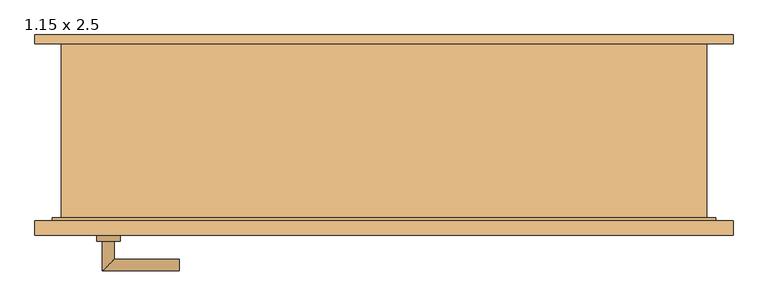
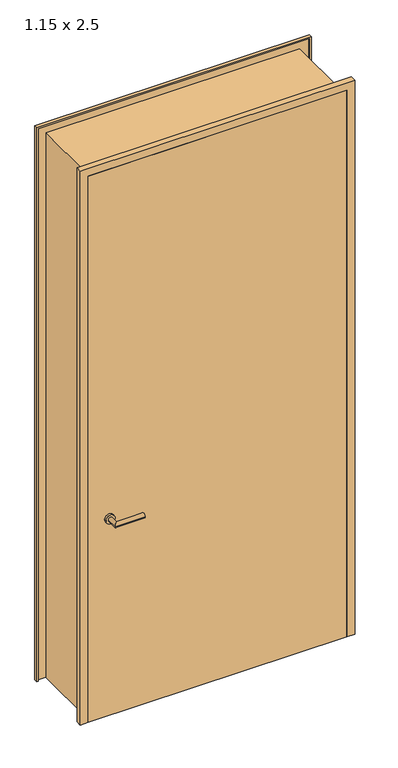
"""IFC4 building model written with IfcOpenShell, lengths in millimetres: door geometry, Drehflügel 1-flg - Stahlzarge : 1.15 x 2.5."""

import ifcopenshell
import ifcopenshell.guid

model = None  # the IFC model being written
_history = None  # IfcOwnerHistory: only IFC2X3 demands one
_inside = {}  # id of a spatial element -> (the spatial element, [elements in it])
_under = {}  # id of a project, library or spatial element -> (it, [spatial elements below it])
_declared = {}  # id of a project -> (the project, [libraries it declares])
_typed = {}  # id of a type object -> (the type object, [elements of that type])
_made_of = {}  # id of a material, layer set ... -> (it, [elements and type objects made of it])


def new_model(schema):
    """Start an empty IFC model of exactly this schema.

    Asked for "IFC4X3", IfcOpenShell would pick the latest addendum, in which some entities
    have other attributes; the version numbers below select the first issue.
    IFC2X3 requires an IfcOwnerHistory on every rooted entity: one is made here for all.
    """
    global model, _history
    if schema == "IFC4X3":
        model = ifcopenshell.file(schema_version=(4, 3, 0, 0))
    else:
        model = ifcopenshell.file(schema=schema)
    _inside.clear()
    _under.clear()
    _declared.clear()
    _typed.clear()
    _made_of.clear()
    _history = None
    if model.schema == "IFC2X3":
        org = make("IfcOrganization", Name="unknown")
        user = make(
            "IfcPersonAndOrganization",
            ThePerson=make("IfcPerson", FamilyName="unknown"),
            TheOrganization=org,
        )
        app = make(
            "IfcApplication",
            ApplicationDeveloper=org,
            Version="unknown",
            ApplicationFullName="unknown",
            ApplicationIdentifier="unknown",
        )
        _history = make(
            "IfcOwnerHistory",
            OwningUser=user,
            OwningApplication=app,
            ChangeAction="ADDED",
            CreationDate=0,
        )
    return model


def make(cls, **values):
    """One entity of the class cls with the attributes given. An attribute that is None is left unset."""
    return model.create_entity(
        cls, **{name: value for name, value in values.items() if value is not None}
    )


def rooted(cls, **values):
    """An entity with a GlobalId (a new one), such as an element, a storey or a relation."""
    return make(cls, GlobalId=ifcopenshell.guid.new(), OwnerHistory=_history, **values)


def si_unit(unit_type, name, prefix=None):
    """IfcSIUnit, for example si_unit("LENGTHUNIT", "METRE", prefix="MILLI")."""
    return make("IfcSIUnit", UnitType=unit_type, Prefix=prefix, Name=name)


def assignment(units):
    """IfcUnitAssignment: the units of a project."""
    return None if units is None else make("IfcUnitAssignment", Units=units)


def point(xyz):
    """IfcCartesianPoint."""
    return None if xyz is None else make("IfcCartesianPoint", Coordinates=xyz)


def direction(xyz):
    """IfcDirection."""
    return None if xyz is None else make("IfcDirection", DirectionRatios=xyz)


def frame(location, z_axis=None, x_axis=None):
    """IfcAxis2Placement3D, a coordinate frame: its origin and axes. An axis left out is left unset."""
    return make(
        "IfcAxis2Placement3D",
        Location=point(location),
        Axis=direction(z_axis),
        RefDirection=direction(x_axis),
    )


def frame_2d(location, x_axis=None):
    """IfcAxis2Placement2D, a coordinate frame in the plane: its origin and x axis."""
    return make(
        "IfcAxis2Placement2D", Location=point(location), RefDirection=direction(x_axis)
    )


def origin():
    """The frame at (0, 0, 0) with its axes left unset."""
    return frame((0.0, 0.0, 0.0))


def place(relative_to, where):
    """IfcLocalPlacement: puts the frame where relative to a parent placement (None: the world)."""
    return make(
        "IfcLocalPlacement", PlacementRelTo=relative_to, RelativePlacement=where
    )


def context(
    kind, dimensions, precision=None, world=None, true_north=None, identifier=None
):
    """IfcGeometricRepresentationContext, for example the 3D "Model" context."""
    return make(
        "IfcGeometricRepresentationContext",
        ContextIdentifier=identifier,
        ContextType=kind,
        CoordinateSpaceDimension=dimensions,
        Precision=precision,
        WorldCoordinateSystem=world,
        TrueNorth=true_north,
    )


def project(units=None, contexts=None):
    """IfcProject with its units and contexts."""
    return rooted(
        "IfcProject",
        Name="project",
        RepresentationContexts=contexts,
        UnitsInContext=assignment(units),
    )


def spatial(cls, under=None, at=None, **own):
    """A site, building, storey or space (cls), placed at a placement, below another one or the project."""
    s = rooted(cls, ObjectPlacement=at, **own)
    if under is not None:
        _under.setdefault(under.id(), (under, []))[1].append(s)
    return s


def polyline(points):
    """IfcPolyline through the points."""
    return make("IfcPolyline", Points=[point(p) for p in points])


def circle_curve(where, radius):
    """IfcCircle in the frame where."""
    return make("IfcCircle", Position=where, Radius=radius)


def ellipse_curve(where, semi_axis1, semi_axis2):
    """IfcEllipse in the frame where."""
    return make(
        "IfcEllipse", Position=where, SemiAxis1=semi_axis1, SemiAxis2=semi_axis2
    )


def trimmed(basis, trim1, trim2, sense, master):
    """IfcTrimmedCurve: the piece of a basis curve between two trims."""
    return make(
        "IfcTrimmedCurve",
        BasisCurve=basis,
        Trim1=trim1,
        Trim2=trim2,
        SenseAgreement=sense,
        MasterRepresentation=master,
    )


def segment(curve, same_sense, transition):
    """IfcCompositeCurveSegment."""
    return make(
        "IfcCompositeCurveSegment",
        Transition=transition,
        SameSense=same_sense,
        ParentCurve=curve,
    )


def composite_curve(segments, self_intersect=None):
    """IfcCompositeCurve: segments joined end to end."""
    return make("IfcCompositeCurve", Segments=segments, SelfIntersect=self_intersect)


def outline(outer, holes=None, kind="AREA"):
    """IfcArbitraryClosedProfileDef: a profile drawn as a closed curve; with holes, ...WithVoids."""
    if holes is None:
        return make("IfcArbitraryClosedProfileDef", ProfileType=kind, OuterCurve=outer)
    return make(
        "IfcArbitraryProfileDefWithVoids",
        ProfileType=kind,
        OuterCurve=outer,
        InnerCurves=holes,
    )


def extrude(swept, where, along, depth):
    """IfcExtrudedAreaSolid: the profile swept, set in the frame where, extruded along a direction by depth."""
    return make(
        "IfcExtrudedAreaSolid",
        SweptArea=swept,
        Position=where,
        ExtrudedDirection=direction(along),
        Depth=depth,
    )


def faces_of(points, faces, orient=None, outer=None):
    """IfcFace entities. A face is a list of loops; a loop is a list of indices into points, from 0.

    orient and outer hold one flag for each loop. By default every Orientation is true, the
    first loop of a face is its IfcFaceOuterBound and the others are IfcFaceBound.
    """
    made = []
    for i, loops in enumerate(faces):
        bounds = []
        for j, loop in enumerate(loops):
            is_outer = j == 0 if outer is None else outer[i][j]
            bounds.append(
                make(
                    "IfcFaceOuterBound" if is_outer else "IfcFaceBound",
                    Bound=make("IfcPolyLoop", Polygon=[points[k] for k in loop]),
                    Orientation=True if orient is None else orient[i][j],
                )
            )
        made.append(make("IfcFace", Bounds=bounds))
    return made


def faceted_brep(points, faces, orient=None, outer=None, voids=None):
    """IfcFacetedBrep: a solid bounded by flat faces; with voids (closed shells), ...WithVoids."""
    shared = [point(p) for p in points]
    hull = make("IfcClosedShell", CfsFaces=faces_of(shared, faces, orient, outer))
    if voids is None:
        return make("IfcFacetedBrep", Outer=hull)
    return make(
        "IfcFacetedBrepWithVoids",
        Outer=hull,
        Voids=[
            make(cls, CfsFaces=faces_of(shared, fs, o, b)) for cls, fs, o, b in voids
        ],
    )


def shape(context_of_items, identifier, shape_type, items):
    """IfcShapeRepresentation: the items that make up one representation, for example the "Body"."""
    return make(
        "IfcShapeRepresentation",
        ContextOfItems=context_of_items,
        RepresentationIdentifier=identifier,
        RepresentationType=shape_type,
        Items=items,
    )


def source(mapping_origin, context_of_items, identifier, shape_type, items):
    """IfcRepresentationMap: a shape defined once, which mapped items show again and again."""
    return make(
        "IfcRepresentationMap",
        MappingOrigin=mapping_origin,
        MappedRepresentation=shape(context_of_items, identifier, shape_type, items),
    )


def transform(
    local_origin,
    x_axis=None,
    y_axis=None,
    z_axis=None,
    scale=None,
    scale2=None,
    scale3=None,
    uniform=True,
):
    """IfcCartesianTransformationOperator3D, or its non-uniform kind. x_axis, y_axis, z_axis: its Axis1, 2, 3."""
    if uniform:
        return make(
            "IfcCartesianTransformationOperator3D",
            Axis1=direction(x_axis),
            Axis2=direction(y_axis),
            LocalOrigin=point(local_origin),
            Scale=scale,
            Axis3=direction(z_axis),
        )
    return make(
        "IfcCartesianTransformationOperator3DnonUniform",
        Axis1=direction(x_axis),
        Axis2=direction(y_axis),
        LocalOrigin=point(local_origin),
        Scale=scale,
        Axis3=direction(z_axis),
        Scale2=scale2,
        Scale3=scale3,
    )


def mapped(mapping_source, mapping_target):
    """IfcMappedItem: shows the shape of a source again, moved by a transform."""
    return make(
        "IfcMappedItem", MappingSource=mapping_source, MappingTarget=mapping_target
    )


def made_of(thing, what):
    """Note that an element or type object is made of a material, layer set ...; save() writes the relation."""
    if what is not None:
        _made_of.setdefault(what.id(), (what, []))[1].append(thing)
    return thing


def element(
    cls,
    number,
    at=None,
    inside=None,
    cuts=None,
    type_object=None,
    material=None,
    context=None,
    identifier="Body",
    shape_type=None,
    held_by="IfcProductDefinitionShape",
    body=None,
    shapes=None,
    **own,
):
    """One element of the class cls, such as IfcWall. Its Tag is "e" and its number.

    at: its placement. inside: the storey or other place that contains it. cuts: it is an
    opening in that element (IfcRelVoidsElement). A single representation is given by context,
    identifier, shape_type and body (its items); several are given by shapes. held_by: the class
    of the entity that holds the representations. save() writes the other relations.
    """
    e = rooted(cls, Tag="e%d" % number, ObjectPlacement=at, **own)
    if body is not None:
        shapes = [shape(context, identifier, shape_type, body)]
    if shapes is not None:
        e.Representation = make(held_by, Representations=shapes)
    if inside is not None:
        _inside.setdefault(inside.id(), (inside, []))[1].append(e)
    if cuts is not None:
        rooted(
            "IfcRelVoidsElement", RelatingBuildingElement=cuts, RelatedOpeningElement=e
        )
    if type_object is not None:
        _typed.setdefault(type_object.id(), (type_object, []))[1].append(e)
    return made_of(e, material)


def aggregate(whole, parts):
    """IfcRelAggregates: a whole, such as a stair, and the parts it consists of."""
    return rooted("IfcRelAggregates", RelatingObject=whole, RelatedObjects=parts)


def save(model, path):
    """Write the relations noted so far, then the file.

    IfcRelAggregates (storeys below a building ...), IfcRelContainedInSpatialStructure (elements
    in a storey), IfcRelDefinesByType, IfcRelAssociatesMaterial and IfcRelDeclares: one each for
    every whole, place, type object, material and project.
    """
    for whole, parts in _under.values():
        aggregate(whole, parts)
    for where, things in _inside.values():
        rooted(
            "IfcRelContainedInSpatialStructure",
            RelatedElements=things,
            RelatingStructure=where,
        )
    for kind, things in _typed.values():
        rooted("IfcRelDefinesByType", RelatedObjects=things, RelatingType=kind)
    for what, things in _made_of.values():
        rooted("IfcRelAssociatesMaterial", RelatedObjects=things, RelatingMaterial=what)
    for by, libraries in _declared.values():
        rooted("IfcRelDeclares", RelatingContext=by, RelatedDefinitions=libraries)
    model.write(path)


def plane_surface(at):
    """IfcPlane: the flat surface through the origin of the frame at, square to its z axis."""
    return make("IfcPlane", Position=at)


def cylinder_surface(at, radius):
    """IfcCylindricalSurface: all points at the distance radius from the z axis of the frame at."""
    return make("IfcCylindricalSurface", Position=at, Radius=radius)


def advanced_brep(points, edges, surfaces, faces):
    """IfcAdvancedBrep: a solid bounded by faces that lie on surfaces and meet in shared edges.

    An edge is (start, end): straight between two places in points (the first is 0);
    or (start, end, curve); or (start, end, curve, False) where it runs against its curve.
    A face is (place in surfaces, loops), or (place, loops, False) where it looks against
    its surface's normal. A loop lists edges by number (the first is 1), with a minus sign
    where the edge is run from its end to its start. The first loop is the outer one.
    """
    corners = [point(p) for p in points]
    vertices = [make("IfcVertexPoint", VertexGeometry=c) for c in corners]
    made = []
    for start, end, *more in edges:
        made.append(
            make(
                "IfcEdgeCurve",
                EdgeStart=vertices[start],
                EdgeEnd=vertices[end],
                EdgeGeometry=more[0] if more else make("IfcPolyline", Points=[corners[start], corners[end]]),
                SameSense=more[1] if len(more) > 1 else True,
            )
        )
    hull = []
    for where, loops, *sense in faces:
        bounds = []
        for j, loop in enumerate(loops):
            ring = [make("IfcOrientedEdge", EdgeElement=made[abs(k) - 1], Orientation=k > 0) for k in loop]
            bounds.append(
                make(
                    "IfcFaceOuterBound" if j == 0 else "IfcFaceBound",
                    Bound=make("IfcEdgeLoop", EdgeList=ring),
                    Orientation=True,
                )
            )
        hull.append(make("IfcAdvancedFace", Bounds=bounds, FaceSurface=surfaces[where], SameSense=sense[0] if sense else True))
    return make("IfcAdvancedBrep", Outer=make("IfcClosedShell", CfsFaces=hull))


def door_1_15_x_2_5_3822d9ce(model_context):
    return source(origin(), model_context, "Body", "SolidModel", [
        advanced_brep(
        [(-477.5, -139.4346141, 901.0), (-457.5, -139.4346141, 901.0), (-457.5, -89.4346141, 901.0), (-477.5, -69.4346141, 901.0), (-347.5, -69.4346141, 901.0), (-347.5, -89.4346141, 901.0)],
        [
            (0, 1, circle_curve(frame((-467.5, -139.4346141, 901.0), z_axis=(0.0, -1.0, 0.0), x_axis=(1.0, 0.0, 0.0)), 10.0)),
            (1, 0, circle_curve(frame((-467.5, -139.4346141, 901.0), z_axis=(0.0, -1.0, 0.0), x_axis=(1.0, 0.0, 0.0)), 10.0)),
            (1, 2),
            (2, 3, ellipse_curve(frame((-467.5, -79.4346141, 901.0), z_axis=(-0.7071067811865385, -0.7071067811865565, 0.0), x_axis=(0.7071067811865563, -0.7071067811865386, 0.0)), 14.1421356, 10.0)),
            (3, 0),
            (3, 2, ellipse_curve(frame((-467.5, -79.4346141, 901.0), z_axis=(-0.7071067811865385, -0.7071067811865565, 0.0), x_axis=(0.7071067811865563, -0.7071067811865386, 0.0)), 14.1421356, 10.0)),
            (4, 5, circle_curve(frame((-347.5, -79.4346141, 901.0), z_axis=(1.0, 0.0, 0.0), x_axis=(0.0, -1.0, 0.0)), 10.0)),
            (5, 4, circle_curve(frame((-347.5, -79.4346141, 901.0), z_axis=(1.0, 0.0, 0.0), x_axis=(0.0, -1.0, 0.0)), 10.0)),
            (2, 5),
            (4, 3),
        ],
        [
            plane_surface(frame((-467.5, -139.4346141, -386.7526403), z_axis=(0.0, -1.0, 0.0), x_axis=(0.0, 0.0, 1.0))),
            cylinder_surface(frame((-467.5, -139.4346141, 901.0), z_axis=(0.0, -1.0, 0.0), x_axis=(1.0, 0.0, 0.0)), 10.0),
            plane_surface(frame((-347.5, -79.4346141, -386.7526403), z_axis=(1.0, 0.0, 0.0), x_axis=(0.0, 0.0, 1.0))),
            cylinder_surface(frame((-467.5, -79.4346141, 901.0), z_axis=(-1.0, 0.0, 0.0), x_axis=(0.0, -1.0, 0.0)), 10.0),
        ],
        [
            (0, [[1, 2]]),
            (1, [[3, 4, 5, -2]]),
            (1, [[-5, 6, -3, -1]]),
            (2, [[7, 8]]),
            (3, [[9, -7, 10, -4]]),
            (3, [[-10, -8, -9, -6]]),
        ],
    ),
        advanced_brep(
        [(-457.5, -199.4346141, 901.0), (-477.5, -199.4346141, 901.0), (-477.5, -249.4346141, 901.0), (-457.5, -229.4346141, 901.0), (-347.5, -229.4346141, 901.0), (-347.5, -249.4346141, 901.0)],
        [
            (0, 1, circle_curve(frame((-467.5, -199.4346141, 901.0), z_axis=(0.0, 1.0, 0.0), x_axis=(-1.0, 0.0, 0.0)), 10.0)),
            (1, 0, circle_curve(frame((-467.5, -199.4346141, 901.0), z_axis=(0.0, 1.0, 0.0), x_axis=(-1.0, 0.0, 0.0)), 10.0)),
            (1, 2),
            (2, 3, ellipse_curve(frame((-467.5, -239.4346141, 901.0), z_axis=(-0.7071067811865475, 0.7071067811865475, 0.0), x_axis=(0.7071067811865474, 0.7071067811865476, 0.0)), 14.1421356, 10.0)),
            (3, 0),
            (3, 2, ellipse_curve(frame((-467.5, -239.4346141, 901.0), z_axis=(-0.7071067811865475, 0.7071067811865475, 0.0), x_axis=(0.7071067811865474, 0.7071067811865476, 0.0)), 14.1421356, 10.0)),
            (4, 5, circle_curve(frame((-347.5, -239.4346141, 901.0), z_axis=(1.0, 0.0, 0.0), x_axis=(0.0, -1.0, 0.0)), 10.0)),
            (5, 4, circle_curve(frame((-347.5, -239.4346141, 901.0), z_axis=(1.0, 0.0, 0.0), x_axis=(0.0, -1.0, 0.0)), 10.0)),
            (2, 5),
            (4, 3),
        ],
        [
            plane_surface(frame((-467.5, -199.4346141, -386.7526403), z_axis=(0.0, 1.0, 0.0), x_axis=(0.0, 0.0, 1.0))),
            cylinder_surface(frame((-467.5, -199.4346141, 901.0), z_axis=(0.0, 1.0, 0.0), x_axis=(-1.0, 0.0, 0.0)), 10.0),
            plane_surface(frame((-347.5, -239.4346141, -386.7526403), z_axis=(1.0, 0.0, 0.0), x_axis=(0.0, 0.0, 1.0))),
            cylinder_surface(frame((-467.5, -239.4346141, 901.0), z_axis=(-1.0, 0.0, 0.0), x_axis=(0.0, -1.0, 0.0)), 10.0),
        ],
        [
            (0, [[1, 2]]),
            (1, [[3, 4, 5, -2]]),
            (1, [[-5, 6, -3, -1]]),
            (2, [[7, 8]]),
            (3, [[9, -7, 10, -4]]),
            (3, [[-10, -8, -9, -6]]),
        ],
    ),
        extrude(outline(composite_curve([segment(trimmed(circle_curve(frame_2d((901.0, -467.5)), 20.0), [point((901.0, -487.5))], [point((901.0, -447.5))], False, "CARTESIAN"), True, "CONTINUOUS"), segment(trimmed(circle_curve(frame_2d((901.0, -467.5)), 20.0), [point((901.0, -447.5))], [point((901.0, -487.5))], False, "CARTESIAN"), True, "CONTINUOUS")], self_intersect=False)), frame((0.0, -139.4346141, 0.0), z_axis=(0.0, 1.0, 0.0), x_axis=(0.0, 0.0, 1.0)), (0.0, 0.0, 1.0), 10.0),
        extrude(outline(composite_curve([segment(trimmed(circle_curve(frame_2d((901.0, -467.5)), 20.0), [point((901.0, -487.5))], [point((901.0, -447.5))], False, "CARTESIAN"), True, "CONTINUOUS"), segment(trimmed(circle_curve(frame_2d((901.0, -467.5)), 20.0), [point((901.0, -447.5))], [point((901.0, -487.5))], False, "CARTESIAN"), True, "CONTINUOUS")], self_intersect=False)), frame((0.0, -199.4346141, 0.0), z_axis=(0.0, 1.0, 0.0), x_axis=(0.0, 0.0, 1.0)), (0.0, 0.0, 1.0), 10.0),
        extrude(outline(polyline([(557.5, -164.4346141), (557.5, -189.4346141), (-557.5, -189.4346141), (-557.5, -164.4346141), (557.5, -164.4346141)])), frame((0.0, 0.0, 1.0), z_axis=(0.0, 0.0, 1.0), x_axis=(1.0, 0.0, 0.0)), (0.0, 0.0, 1.0), 2490.0),
        faceted_brep([(591.9603207, 150.5653859, 1.0), (591.9603207, 135.5653859, 1.0), (586.9603207, 135.5653859, 1.0), (586.9603207, 145.5653859, 1.0), (547.5, 145.5653859, 1.0), (547.5, -159.4346141, 1.0), (562.5, -159.4346141, 1.0), (562.5, -184.4346141, 1.0), (586.9603207, -184.4346141, 1.0), (586.9603207, -164.4346141, 1.0), (591.9603207, -164.4346141, 1.0), (591.9603207, -189.4346141, 1.0), (557.5, -189.4346141, 1.0), (557.5, -164.4346141, 1.0), (542.5, -164.4346141, 1.0), (542.5, 150.5653859, 1.0), (542.5, 150.5653859, 2476.0), (-542.5, 150.5653859, 2476.0), (-542.5, 150.5653859, 1.0), (-591.9603207, 150.5653859, 1.0), (-591.9603207, 150.5653859, 2525.4603207), (591.9603207, 150.5653859, 2525.4603207), (542.5, -164.4346141, 2476.0), (557.5, -164.4346141, 2491.0), (-557.5, -164.4346141, 2491.0), (-557.5, -164.4346141, 1.0), (-542.5, -164.4346141, 1.0), (-542.5, -164.4346141, 2476.0), (557.5, -189.4346141, 2491.0), (591.9603207, -189.4346141, 2525.4603207), (-591.9603207, -189.4346141, 2525.4603207), (-591.9603207, -189.4346141, 1.0), (-557.5, -189.4346141, 1.0), (-557.5, -189.4346141, 2491.0), (591.9603207, -164.4346141, 2525.4603207), (586.9603207, -164.4346141, 2520.4603207), (-586.9603207, -164.4346141, 2520.4603207), (-586.9603207, -164.4346141, 1.0), (-591.9603207, -164.4346141, 1.0), (-591.9603207, -164.4346141, 2525.4603207), (586.9603207, -184.4346141, 2520.4603207), (562.5, -184.4346141, 2496.0), (-562.5, -184.4346141, 2496.0), (-562.5, -184.4346141, 1.0), (-586.9603207, -184.4346141, 1.0), (-586.9603207, -184.4346141, 2520.4603207), (562.5, -159.4346141, 2496.0), (547.5, -159.4346141, 2481.0), (-547.5, -159.4346141, 2481.0), (-547.5, -159.4346141, 1.0), (-562.5, -159.4346141, 1.0), (-562.5, -159.4346141, 2496.0), (547.5, 145.5653859, 2481.0), (586.9603207, 145.5653859, 2520.4603207), (-586.9603207, 145.5653859, 2520.4603207), (-586.9603207, 145.5653859, 1.0), (-547.5, 145.5653859, 1.0), (-547.5, 145.5653859, 2481.0), (586.9603207, 135.5653859, 2520.4603207), (591.9603207, 135.5653859, 2525.4603207), (-591.9603207, 135.5653859, 2525.4603207), (-591.9603207, 135.5653859, 1.0), (-586.9603207, 135.5653859, 1.0), (-586.9603207, 135.5653859, 2520.4603207)], [[[0, 1, 2, 3, 4, 5, 6, 7, 8, 9, 10, 11, 12, 13, 14, 15]], [[15, 16, 17, 18, 19, 20, 21, 0]], [[14, 22, 16, 15]], [[13, 23, 24, 25, 26, 27, 22, 14]], [[12, 28, 23, 13]], [[11, 29, 30, 31, 32, 33, 28, 12]], [[10, 34, 29, 11]], [[9, 35, 36, 37, 38, 39, 34, 10]], [[8, 40, 35, 9]], [[7, 41, 42, 43, 44, 45, 40, 8]], [[6, 46, 41, 7]], [[5, 47, 48, 49, 50, 51, 46, 6]], [[4, 52, 47, 5]], [[3, 53, 54, 55, 56, 57, 52, 4]], [[2, 58, 53, 3]], [[1, 59, 60, 61, 62, 63, 58, 2]], [[0, 21, 59, 1]], [[20, 19, 61, 60]], [[19, 18, 26, 25, 32, 31, 38, 37, 44, 43, 50, 49, 56, 55, 62, 61]], [[27, 26, 18, 17]], [[33, 32, 25, 24]], [[39, 38, 31, 30]], [[45, 44, 37, 36]], [[51, 50, 43, 42]], [[57, 56, 49, 48]], [[63, 62, 55, 54]], [[22, 27, 17, 16]], [[28, 33, 24, 23]], [[34, 39, 30, 29]], [[40, 45, 36, 35]], [[46, 51, 42, 41]], [[52, 57, 48, 47]], [[58, 63, 54, 53]], [[21, 20, 60, 59]]]),
    ])


if __name__ == "__main__":
    model = new_model("IFC4")
    model_context = context("Model", 3, world=origin())
    ifc_project = project(units=[si_unit("LENGTHUNIT", "METRE", prefix="MILLI")], contexts=[model_context])
    site = spatial("IfcSite", under=ifc_project)
    building = spatial("IfcBuilding", under=site)
    placement = place(None, origin())
    door_1_15_x_2_5_shape = door_1_15_x_2_5_3822d9ce(model_context)
    element("IfcDoor", 1, ObjectType="Drehflügel 1-flg - Stahlzarge : 1.15 x 2.5", at=placement, inside=building, context=model_context, shape_type="MappedRepresentation", body=[
        mapped(door_1_15_x_2_5_shape, transform((0.0, 0.0, 0.0), x_axis=(1.0, 0.0, 0.0), y_axis=(0.0, 1.0, 0.0), z_axis=(0.0, 0.0, 1.0))),
    ])
    save(model, "model.ifc")

# Revit data of these elements
# Type "Drehflügel 1-flg - Stahlzarge : 1.15 x 2.5"
#   Type Mark = "21"
#   Operation = "SingleSwingRight"
#   Keynote = "16.03"
#   Analytic Construction = "Metall"
#   Thermal Resistance (R) = 0.270117 (m²·K)/W
#   Heat Transfer Coefficient (U) = 3.7021 W/(m²·K)
#   Rough Width = 1.135 m
#   Rough Height [instance default] = 2.600 m
#   Höhe Türgriff [instance default] = 0.900 m
#   Height = 2.500 m
#   Fußbodenaufbau [instance default] = 0.100 m
#   Width = 1.135 m
#   Sichtbarkeit Sturzlinien [instance default] = yes
#   Türgriff auswählen [instance default] = element 221079
#   Türgriff [instance default] = none
#   Türflügel [instance default] = none
#   Rahmen/Pfosten [instance default] = Metall - Lackiert - Grau
#   Visual Light Transmittance = 0
#   Solar Heat Gain Coefficient = 0
#   Function = (empty or 0)
#   Wall Closure = (empty or 0)
# Element 1 (IfcDoor, "Drehflügel 1-flg - Stahlzarge : 1.15 x 2.5")
#   Rough Height = 2.501 m
#   Fußbodenaufbau = 0.001 m
#   Materials on its faces: "Metall - Lackiert - Grau", "Metall - Chrom", "Holz - Birke"
# Materials
#   "Metall - Lackiert - Grau": class "Farbe 1", colour RGB 98 98 98, transparency 0, Cost = 0
#   "Metall - Chrom": class "Metall", colour RGB 247 247 247, transparency 0, Cost = 0
#   "Holz - Birke": class "Holz", colour RGB 213 164 103, transparency 0, Cost = 0
